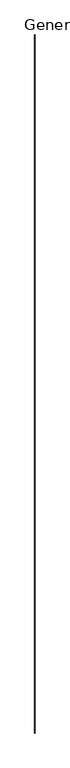
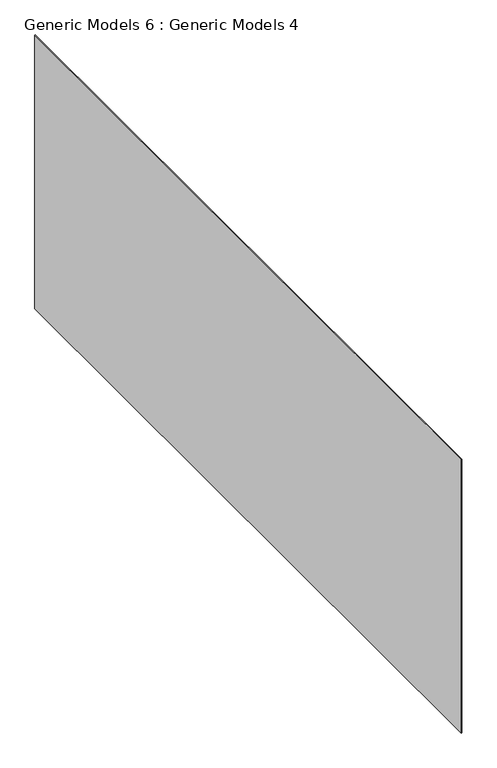
"""IFC4 building model written with IfcOpenShell, lengths in millimetres: proxy geometry, Generic Models 6 : Generic Models 4."""

from ifc_helpers import new_model, si_unit, frame, origin, place, context, project, spatial, polyline, outline, extrude, source, transform, mapped, element, save


def generic_models_6_generic_models_4_ff3d2fe5(model_context):
    return source(origin(), model_context, "Body", "SweptSolid", [
        extrude(outline(polyline([(570255.1076893, -527524.3545647), (570255.1076893, -584979.050959), (570229.7076893, -584979.050959), (570229.7076893, -527524.3545647), (570255.1076893, -527524.3545647)])), frame((0.0, 0.0, -2503.337634), z_axis=(0.0, 0.0, 1.0), x_axis=(1.0, 0.0, 0.0)), (0.0, 0.0, 1.0), 22488.6259865),
    ])


if __name__ == "__main__":
    model = new_model("IFC4")
    model_context = context("Model", 3, world=origin())
    ifc_project = project(units=[si_unit("LENGTHUNIT", "METRE", prefix="MILLI")], contexts=[model_context])
    site = spatial("IfcSite", under=ifc_project)
    building = spatial("IfcBuilding", under=site)
    placement = place(None, origin())
    generic_models_6_generic_models_4_shape = generic_models_6_generic_models_4_ff3d2fe5(model_context)
    element("IfcBuildingElementProxy", 1, Name="Generic Models 6 : Generic Models 4", ObjectType="Generic Models 6 : Generic Models 4", at=placement, inside=building, context=model_context, shape_type="MappedRepresentation", body=[
        mapped(generic_models_6_generic_models_4_shape, transform((0.0, 0.0, 0.0), x_axis=(1.0, 0.0, 0.0), y_axis=(0.0, 1.0, 0.0), z_axis=(0.0, 0.0, 1.0))),
    ])
    save(model, "model.ifc")

# Revit data of these elements
# Element 1 (IfcBuildingElementProxy, "Generic Models 6 : Generic Models 4")
#   Materials on its faces: "Air"
# Materials
#   "Air": class "Gas", colour RGB 255 255 255, transparency 1, Description = "Air", Cost = 0
